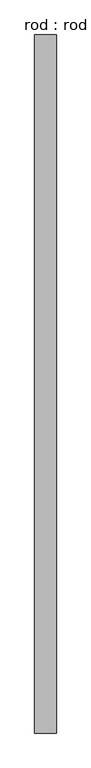
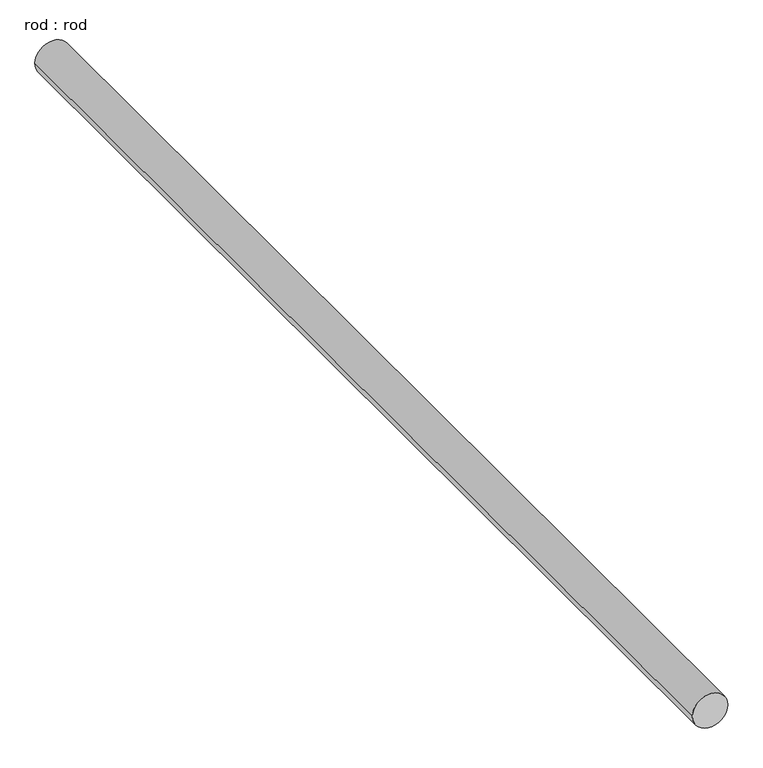
"""IFC4 building model written with IfcOpenShell, lengths in millimetres: proxy geometry, rod : rod."""

from ifc_helpers import new_model, si_unit, point, frame, frame_2d, origin, place, context, project, spatial, circle_curve, trimmed, segment, composite_curve, outline, extrude, source, transform, mapped, element, save


def rod_rod_c746abc9(model_context):
    return source(origin(), model_context, "Body", "SweptSolid", [
        extrude(outline(composite_curve([segment(trimmed(circle_curve(frame_2d((0.0108462, 0.0)), 200.0), [point((0.0108462, 200.0))], [point((0.0108462, -200.0))], False, "CARTESIAN"), True, "CONTINUOUS"), segment(trimmed(circle_curve(frame_2d((0.0108462, 0.0)), 200.0), [point((0.0108462, -200.0))], [point((0.0108462, 200.0))], False, "CARTESIAN"), True, "CONTINUOUS")], self_intersect=False)), frame((0.0, -2359.4996819, 0.0), z_axis=(0.0, 1.0, 0.0), x_axis=(0.0, 0.0, 1.0)), (0.0, 0.0, 1.0), 12904.4565945),
    ])


if __name__ == "__main__":
    model = new_model("IFC4")
    model_context = context("Model", 3, world=origin())
    ifc_project = project(units=[si_unit("LENGTHUNIT", "METRE", prefix="MILLI")], contexts=[model_context])
    site = spatial("IfcSite", under=ifc_project)
    building = spatial("IfcBuilding", under=site)
    placement = place(None, origin())
    rod_rod_shape = rod_rod_c746abc9(model_context)
    element("IfcBuildingElementProxy", 1, Name="rod : rod", ObjectType="rod : rod", at=placement, inside=building, context=model_context, shape_type="MappedRepresentation", body=[
        mapped(rod_rod_shape, transform((0.0, 0.0, 0.0), x_axis=(1.0, 0.0, 0.0), y_axis=(0.0, 1.0, 0.0), z_axis=(0.0, 0.0, 1.0))),
    ])
    save(model, "model.ifc")

# Revit data of these elements
# Type "rod : rod"
#   Default Elevation = 0
